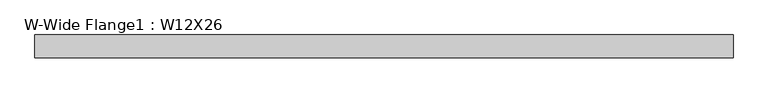
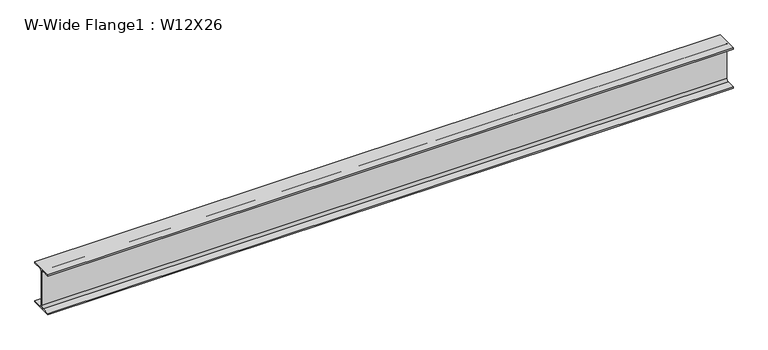
"""IFC4 building model written with IfcOpenShell, lengths in millimetres: beam geometry, W-Wide Flange1 : W12X26."""

from ifc_helpers import new_model, si_unit, point, frame, frame_2d, origin, place, context, project, spatial, polyline, circle_curve, trimmed, segment, composite_curve, outline, extrude, source, transform, mapped, element, save


def w_wide_flange1_w12x26_895a7735(model_context):
    return source(origin(), model_context, "Body", "SweptSolid", [
        extrude(outline(composite_curve([segment(polyline([(82.423, -145.288), (82.423, -154.94), (-82.423, -154.94), (-82.423, -145.288), (-20.2565, -145.288)]), True, "CONTINUOUS"), segment(trimmed(circle_curve(frame_2d((-20.2565, -127.9525)), 17.3355), [point((-20.2565, -145.288))], [point((-2.921, -127.9525))], True, "CARTESIAN"), True, "CONTINUOUS"), segment(polyline([(-2.921, -127.9525), (-2.921, 127.9525)]), True, "CONTINUOUS"), segment(trimmed(circle_curve(frame_2d((-20.2565, 127.9525)), 17.3355), [point((-2.921, 127.9525))], [point((-20.2565, 145.288))], True, "CARTESIAN"), True, "CONTINUOUS"), segment(polyline([(-20.2565, 145.288), (-82.423, 145.288), (-82.423, 154.94), (82.423, 154.94), (82.423, 145.288), (20.2565, 145.288)]), True, "CONTINUOUS"), segment(trimmed(circle_curve(frame_2d((20.2565, 127.9525)), 17.3355), [point((20.2565, 145.288))], [point((2.921, 127.9525))], True, "CARTESIAN"), True, "CONTINUOUS"), segment(polyline([(2.921, 127.9525), (2.921, -127.9525)]), True, "CONTINUOUS"), segment(trimmed(circle_curve(frame_2d((20.2565, -127.9525)), 17.3355), [point((2.921, -127.9525))], [point((20.2565, -145.288))], True, "CARTESIAN"), True, "CONTINUOUS"), segment(polyline([(20.2565, -145.288), (82.423, -145.288)]), True, "CONTINUOUS")], self_intersect=False)), frame((-2496.2512479, 0.0, 0.0), z_axis=(1.0, 0.0, 0.0), x_axis=(0.0, 1.0, 0.0)), (0.0, 0.0, 1.0), 4995.2451716),
    ])


if __name__ == "__main__":
    model = new_model("IFC4")
    model_context = context("Model", 3, world=origin())
    ifc_project = project(units=[si_unit("LENGTHUNIT", "METRE", prefix="MILLI")], contexts=[model_context])
    site = spatial("IfcSite", under=ifc_project)
    building = spatial("IfcBuilding", under=site)
    placement = place(None, origin())
    w_wide_flange1_w12x26_shape = w_wide_flange1_w12x26_895a7735(model_context)
    element("IfcBeam", 1, ObjectType="W-Wide Flange1 : W12X26", at=placement, inside=building, context=model_context, shape_type="MappedRepresentation", body=[
        mapped(w_wide_flange1_w12x26_shape, transform((0.0, 0.0, 0.0), x_axis=(1.0, 0.0, 0.0), y_axis=(0.0, 1.0, 0.0), z_axis=(0.0, 0.0, 1.0))),
    ])
    save(model, "model.ifc")

# Revit data of these elements
# Type "W-Wide Flange1 : W12X26"
#   Assembly Code = "B10"
#   W = 26
#   Start Extension Calculation [instance default] = 10' - 0"
#   Start Extension [instance default] = -0' - 0 1/2"
#   End Extension Calculation [instance default] = 10' - 0"
#   End Extension [instance default] = -0' - 0 1/2"
#   Length [instance default] = 5' - 0"
#   bf = 0' - 6.49"
#   d = 1' - 0.2"
#   k = 0' - 1 1/16"
#   k2 = 0' - 0.6825"
#   tf = 0' - 0.38"
#   tw = 0' - 0.23"
#   A = 0.053125 SF
#   Structural Material [instance default] = Metal - Steel - ASTM A992
# Element 1 (IfcBeam, "W-Wide Flange1 : W12X26")
#   Materials on its faces: "Metal - Steel - ASTM A992"
# Materials
#   "Metal - Steel - ASTM A992": class "Metal", colour RGB 199 199 199, transparency 0
